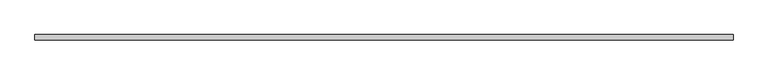
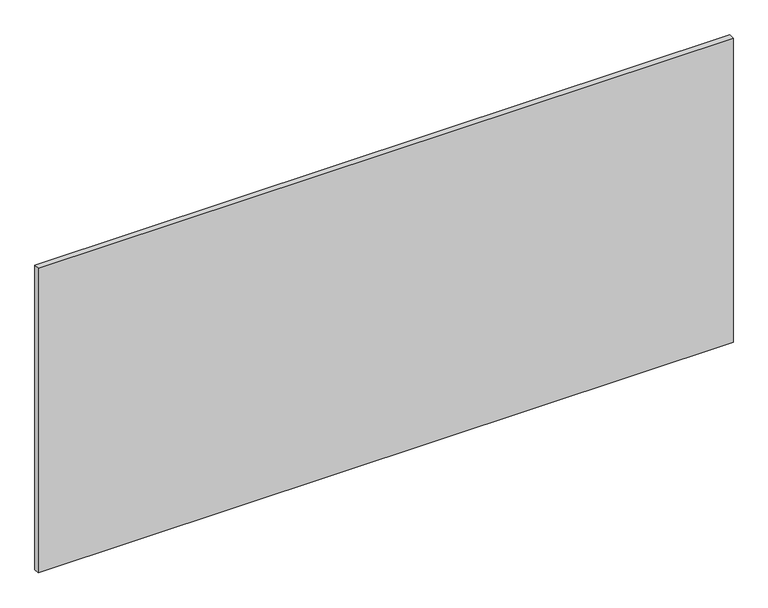
"""IFC4 building model written with IfcOpenShell, lengths in millimetres: proxy geometry, Inner panel:Inner panel:1:Inner panel:1 : Inner panel:Inner panel:300324:300043:Inner panel:1:Inner panel:1 : Inner panel:Inner panel:300324:300043 : Inner panel:Inner panel:1:Inner panel:1 : Inner panel:Inner panel:300324:300043:20 : Inner panel:Inner panel:1:Inner panel:1 : Inner panel:Inner panel:300324:300043:Inner panel:1:Inner panel:1 : Inner panel:Inner panel:300324:300043 : Inner panel:Inner panel:1:Inner panel:1 : Inner panel:Inner panel:300324:300043:300031."""

from ifc_helpers import new_model, si_unit, frame, origin, place, context, project, spatial, polyline, outline, extrude, source, transform, mapped, element, save


def generic_models_310391fb(model_context):
    return source(origin(), model_context, "Body", "SweptSolid", [
        extrude(outline(polyline([(592512.5367239, -568186.6413841), (594950.9367239, -568186.6413841), (594950.9367239, -568205.6913841), (592512.5367239, -568205.6913841), (592512.5367239, -568186.6413841)])), frame((0.0, 0.0, 3721.1), z_axis=(0.0, 0.0, 1.0), x_axis=(1.0, 0.0, 0.0)), (0.0, 0.0, 1.0), 1129.1980526),
    ])


if __name__ == "__main__":
    model = new_model("IFC4")
    model_context = context("Model", 3, world=origin())
    ifc_project = project(units=[si_unit("LENGTHUNIT", "METRE", prefix="MILLI")], contexts=[model_context])
    site = spatial("IfcSite", under=ifc_project)
    building = spatial("IfcBuilding", under=site)
    placement = place(None, origin())
    generic_models_shape = generic_models_310391fb(model_context)
    element("IfcBuildingElementProxy", 1, Name="Inner panel:Inner panel:1:Inner panel:1 : Inner panel:Inner panel:300324:300043:Inner panel:1:Inner panel:1 : Inner panel:Inner panel:300324:300043 : Inner panel:Inner panel:1:Inner panel:1 : Inner panel:Inner panel:300324:300043:20 : Inner panel:Inner panel:1:Inner panel:1 : Inner panel:Inner panel:300324:300043:Inner panel:1:Inner panel:1 : Inner panel:Inner panel:300324:300043 : Inner panel:Inner panel:1:Inner panel:1 : Inner panel:Inner panel:300324:300043:300031", ObjectType="Inner panel:Inner panel:1:Inner panel:1 : Inner panel:Inner panel:300324:300043:Inner panel:1:Inner panel:1 : Inner panel:Inner panel:300324:300043 : Inner panel:Inner panel:1:Inner panel:1 : Inner panel:Inner panel:300324:300043:20 : Inner panel:Inner panel:1:Inner panel:1 : Inner panel:Inner panel:300324:300043:Inner panel:1:Inner panel:1 : Inner panel:Inner panel:300324:300043 : Inner panel:Inner panel:1:Inner panel:1 : Inner panel:Inner panel:300324:300043:300031", at=placement, inside=building, context=model_context, shape_type="MappedRepresentation", body=[
        mapped(generic_models_shape, transform((0.0, 0.0, 0.0), x_axis=(1.0, 0.0, 0.0), y_axis=(0.0, 1.0, 0.0), z_axis=(0.0, 0.0, 1.0))),
    ])
    save(model, "model.ifc")

# Revit data of these elements
# Type "Inner panel:Inner panel:1:Inner panel:1 : Inner panel:Inner panel:300324:300043:Inner panel:1:Inner panel:1 : Inner panel:Inner panel:300324:300043 : Inner panel:Inner panel:1:Inner panel:1 : Inner panel:Inner panel:300324:300043:20 : Inner panel:Inner panel:1:Inner panel:1 : Inner panel:Inner panel:300324:300043:Inner panel:1:Inner panel:1 : Inner panel:Inner panel:300324:300043 : Inner panel:Inner panel:1:Inner panel:1 : Inner panel:Inner panel:300324:300043:300031"
#   NameOverride = "Inner panel:Inner panel:1:Inner panel:1 : Inner panel:Inner panel:300324:300043:Inner panel:1:Inner panel:1 : Inner panel:Inner panel:300324:300043 : Inner panel:Inner panel:1:Inner panel:1 : Inner panel:Inner panel:300324:300043:300031"
#   ObjectTypeOverride = "Inner panel:1:Inner panel:1 : Inner panel:Inner panel:300324:300043 : Inner panel:Inner panel:1:Inner panel:1 : Inner panel:Inner panel:300324:300043"
#   Reference = "Inner panel"
#   Tag = "300031"
# Element 1 (IfcBuildingElementProxy, "Inner panel:Inner panel:1:Inner panel:1 : Inner panel:Inner panel:300324:300043:Inner panel:1:Inner panel:1 : Inner panel:Inner panel:300324:300043 : Inner panel:Inner panel:1:Inner panel:1 : Inner panel:Inner panel:300324:300043:20 : Inner panel:Inner panel:1:Inner panel:1 : Inner panel:Inner panel:300324:300043:Inner panel:1:Inner panel:1 : Inner panel:Inner panel:300324:300043 : Inner panel:Inner panel:1:Inner panel:1 : Inner panel:Inner panel:300324:300043:300031")
#   Materials on its faces: "¾” (CLASS A) FIRE RETARDANT PLYWOOD"
# Materials
#   "¾” (CLASS A) FIRE RETARDANT PLYWOOD": class "Wood", colour RGB 149 120 74, transparency 0, Description = "Plywood, sheathing grade", Cost = 0
